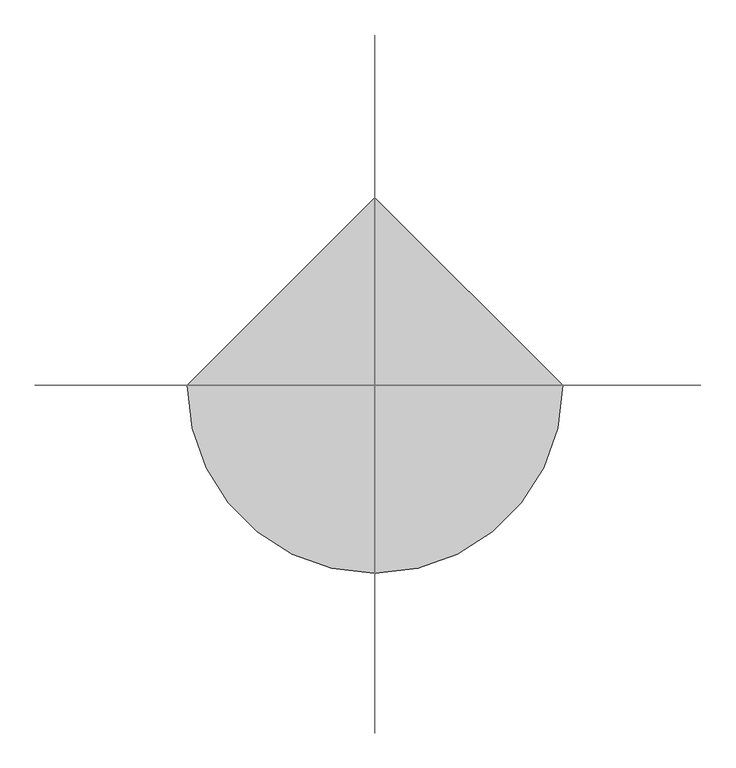
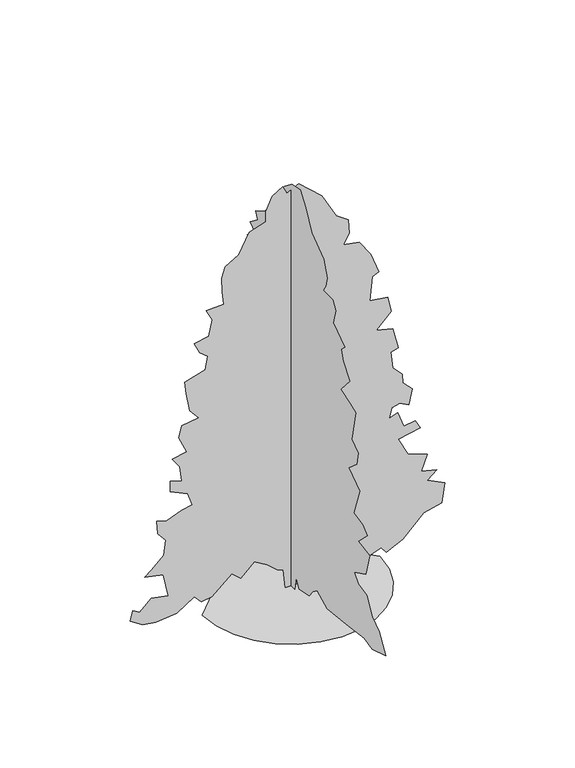
"""IFC4 building model written with IfcOpenShell, lengths in millimetres: proxy geometry, colorado spruce 26066 : colorado spruce 26066."""

from ifc_helpers import new_model, si_unit, origin, place, context, project, spatial, triangles, source, transform, mapped, element, save


def entourage_51173285(model_context):
    return source(origin(), model_context, "Body", "Tessellation", [
        triangles([(2.3e-06, 50.6216921, 3.68e-05), (9.8e-06, 78.1276076, 213.1710181), (1.43e-05, 112.5100566, 309.4405598), (1.77e-05, 236.2865403, 240.6769336), (2.27e-05, 387.5684217, 178.7885601), (2.95e-05, 559.4807118, 151.2826536), (3.74e-05, 731.8705164, 158.5998759), (3.48e-05, 752.0228474, 41.258996), (4.28e-05, 875.7995945, 123.776738), (4.61e-05, 1007.1354006, 36.9163581), (5.13e-05, 1102.7231707, 68.7649115), (5.94e-05, 1288.3895267, 61.888369), (6.59e-05, 1377.7823261, 144.4061111), (8e-05, 1570.324498, 330.0704415), (7.64e-05, 1453.423494, 385.0817639), (7.29e-05, 1350.2767376, 419.465748), (6.83e-05, 1254.1961197, 411.4393484), (7.07e-05, 1233.3757336, 522.6126134), (7.48e-05, 1260.8813221, 618.883663), (8.24e-05, 1357.1524807, 728.9063078), (7.87e-05, 1260.8813221, 749.5362259), (8.41e-05, 1336.5226353, 818.3016506), (7.99e-05, 1219.624102, 852.6830549), (7.62e-05, 1095.8474276, 914.5726639), (7.72e-05, 1032.2102509, 1041.9130743), (8.57e-05, 1192.1185135, 1086.4849903), (9.06e-05, 1260.8813221, 1148.3720558), (8.72e-05, 1171.4885954, 1169.0019739), (8.31e-05, 1020.2061871, 1258.3973167), (8.97e-05, 1130.2288319, 1313.4086391), (9.55e-05, 1139.1290154, 1494.4927895), (9.04e-05, 1013.3279005, 1512.8265541), (8.63e-05, 903.3052557, 1540.3321426), (9.07e-05, 919.5358784, 1665.6252216), (9.79e-05, 1053.5310425, 1703.3976254), (0.0001031, 1082.0933252, 1836.0212162), (9.76e-05, 972.0706804, 1815.3912254), (9.84e-05, 902.5889477, 1949.2238995), (0.0001046, 978.9464235, 2042.3148743), (0.0001028, 882.6754103, 2124.8319305), (0.0001091, 978.9464235, 2193.5973553), (0.000112, 1006.4520847, 2248.6086777), (0.0001076, 834.539831, 2358.6337933), (0.0001087, 813.9099855, 2427.3966019), (0.0001169, 951.4407623, 2496.1621719), (0.0001168, 889.5511534, 2585.5674706), (0.0001125, 752.0228474, 2647.4418915), (0.0001196, 841.4156467, 2750.5914093), (0.0001179, 745.1445608, 2839.9740349), (0.0001151, 621.3703571, 2929.3819496), (0.0001181, 614.4919979, 3039.4147682), (0.0001241, 717.6388996, 3087.5475861), (0.0001224, 642.0002026, 3142.5639954), (0.000119, 552.6049324, 3163.1888992), (0.0001267, 669.5058638, 3245.688224), (0.000124, 545.729153, 3341.9794395), (0.0001276, 580.1105936, 3410.7374519), (0.0001236, 435.7039647, 3493.2617752), (0.000122, 318.802997, 3617.0361969), (0.0001233, 241.6693149, 3775.8113892), (0.000122, 98.7569716, 3947.1090729), (0.0001198, -11.2668813, 4036.4916985), (0.0001145, -148.7964954, 4063.9999031), (0.0001065, -245.067327, 3940.2257721), (9.64e-05, -341.337886, 3747.6936287), (8.32e-05, -540.7558373, 3603.2693047), (7.6e-05, -595.7671597, 3445.1289574), (7.44e-05, -568.2614985, 3348.8374512), (7.41e-05, -533.8800579, 3286.9630302), (6.73e-05, -685.1624662, 3286.9630302), (6.27e-05, -733.2979729, 3204.4384163), (6.03e-05, -692.0382093, 3060.0396721), (4.78e-05, -884.5803812, 2929.3819496), (4.89e-05, -822.6907722, 2874.3655403), (4.43e-05, -857.07472, 2771.2160225), (3.55e-05, -967.0973648, 2640.5585907), (3.71e-05, -815.8149565, 2468.6562927), (2.85e-05, -975.0983299, 2418.8978474), (2.34e-05, -1063.3684507, 2379.2636387), (1.71e-05, -1001.4787691, 2076.6963512), (1.03e-05, -1104.6282143, 2001.0551834), (7.5e-06, -1083.9982962, 1877.2784363), (9.8e-06, -953.3432625, 1760.3800484), (-1.8e-06, -1132.1338755, 1636.6033012), (-5.6e-06, -1028.9869738, 1354.6658592), (-1.32e-05, -1180.2693821, 1327.1601254), (-1.84e-05, -1255.9105499, 1265.2730598), (-1.62e-05, -1104.6282143, 1113.9906515), (-2.56e-05, -1297.16777, 1086.4849903), (-2.93e-05, -1228.4049614, 859.5588707), (-2.37e-05, -1042.7385326, 770.1660713), (-2.89e-05, -1104.6282143, 687.6490877), (-3.62e-05, -1249.032336, 660.1434265), (-4.49e-05, -1338.4276062, 501.9827316), (-5.26e-05, -1455.3284649, 419.465748), (-6.25e-05, -1558.4753666, 240.6769336), (-5.47e-05, -1338.4276062, 171.9120176), (-4.78e-05, -1203.4697828, 202.7582816), (-3.57e-05, -909.8228811, 166.6996904), (-2.27e-05, -595.7671597, 130.6530262), (-1.29e-05, -430.7306491, 213.1710181), (-1.15e-05, -361.9677678, 158.1589326), (-1.1e-05, -300.0781407, 82.5177376), (-4.6e-06, -135.0434104, 48.1355384), (1e-07, -87.2685559, 135.4498173), (-2.7e-06, -59.4022154, 3.35e-05), (-52.2236701, 1.3e-06, 3.68e-05), (-72.8530386, -2.11e-05, 185.6651025), (-127.8648697, -2.04e-05, 206.2944756), (-224.1356831, -2.12e-05, 288.8132396), (-347.9113947, -2.09e-05, 364.4544256), (-478.5664647, 3.3e-06, 240.6769336), (-561.0834483, 2.4e-06, 316.3188827), (-753.6255838, 1.55e-05, 151.2826536), (-850.3106707, 1.89e-05, 139.1823475), (-918.659551, 1.76e-05, 213.1710181), (-1083.6960617, 2.75e-05, 103.147365), (-1283.1139767, 4.91e-05, 82.5179919), (-1406.8907238, 5.18e-05, 103.147365), (-1523.7917278, 5.2e-05, 178.7885601), (-1503.1617371, 4.7e-05, 275.0591373), (-1434.3964577, 4.68e-05, 233.8003911), (-1324.3711967, 2.42e-05, 336.9487644), (-1166.2130453, 2.07e-05, 309.4405598), (-1212.8550385, 1.19e-05, 536.5622706), (-1386.2608784, 1.56e-05, 570.7481564), (-1324.3711967, 1.16e-05, 618.883663), (-1207.4728088, 3.2e-06, 728.9063078), (-1186.8428907, -3.9e-06, 873.312973), (-1262.4841312, -5.6e-06, 962.7082432), (-1276.2382336, -1.11e-05, 1093.3607334), (-1179.9671476, -1.27e-05, 1065.8550722), (-1035.5604824, -3.42e-05, 1120.8663946), (-939.2894691, -3.8e-05, 1141.4963127), (-980.5492327, -4.23e-05, 1265.2730598), (-1145.7305019, -4.09e-05, 1342.6363609), (-1145.5831272, -4.57e-05, 1450.9368725), (-1035.5604824, -4.74e-05, 1416.5553955), (-1054.1152365, -5.34e-05, 1562.7171135), (-1124.9558252, -5.58e-05, 1664.1088898), (-987.4249758, -6.12e-05, 1691.6146236), (-1063.0661436, -6.63e-05, 1856.6484455), (-1035.5604824, -7.2e-05, 1966.6737064), (-877.402331, -9.27e-05, 1994.179295), (-959.9193146, -9.46e-05, 2090.4504536), (-994.3007915, -0.0001019, 2276.1142662), (-1008.0548212, -0.0001067, 2393.0152702), (-815.512722, -0.0001152, 2454.9021904), (-788.0070608, -0.0001215, 2578.6841698), (-863.6482286, -0.000122, 2640.5585907), (-918.659551, -0.0001253, 2750.5914093), (-778.8249178, -0.0001453, 2774.1370651), (-746.7472973, -0.0001532, 2929.3819496), (-801.7586197, -0.0001565, 3039.4147682), (-636.7246525, -0.0001617, 3046.2727798), (-650.4762114, -0.0001671, 3176.9302116), (-657.3544979, -0.0001731, 3314.4712349), (-622.9705502, -0.0001787, 3417.6207527), (-495.5108156, -0.0002008, 3495.9796326), (-396.0469377, -0.0002122, 3685.7939186), (-237.8885137, -0.0002191, 3733.9270271), (-237.8885137, -0.0002237, 3837.0762543), (-176.0001583, -0.0002314, 3967.7339767), (-79.7295811, -0.000237, 4029.6083977), (-38.4705851, -0.0002349, 3953.9670845), (71.553068, -0.0002554, 4008.9834938), (291.5996066, -0.000253, 3809.5680496), (429.1304561, -0.0002313, 3562.0197876), (546.0314238, -0.0002458, 3479.4951736), (552.9072032, -0.0002251, 3341.9794395), (497.8958808, -0.0002192, 3245.688224), (649.1782528, -0.0002225, 3218.2053085), (759.2008976, -0.0002187, 3060.0396721), (834.8420654, -0.000212, 2860.6242279), (772.2870174, -0.0002087, 2828.0866791), (745.4493387, -0.0001977, 2599.3090736), (917.359049, -0.0002016, 2571.800869), (951.7430695, -0.0001958, 2420.5208588), (807.3364769, -0.0001854, 2282.9926254), (965.4946283, -0.0001882, 2241.7327892), (1020.5084942, -0.0001656, 2028.5607719), (944.8647102, -0.0001627, 2014.8092857), (965.4946283, -0.000156, 1849.7727024), (1056.4342083, -0.0001542, 1750.4358879), (1061.7657143, -0.0001505, 1664.1088898), (1151.1609844, -0.0001492, 1574.7136196), (1116.7770367, -0.0001414, 1423.4311386), (1034.2600531, -0.0001411, 1471.5667179), (958.6188126, -0.0001379, 1450.9368725), (931.1131514, -0.0001328, 1354.6658592), (1013.630135, -0.0001365, 1382.1714478), (1068.6414574, -0.0001311, 1224.0132236), (1178.6666456, -0.0001353, 1244.6432144), (1226.8021523, -0.0001327, 1155.2478716), (1020.5084942, -0.0001247, 1113.9906515), (1109.9012209, -0.0001046, 935.2000385), (1295.567577, -0.0001218, 866.4371572), (1236.1544884, -9.85e-05, 715.1572924), (1384.9603764, -0.0001014, 680.7708012), (1295.567577, -9.54e-05, 605.129597), (1460.6015442, -9.66e-05, 522.6126134), (1433.0959557, -8.72e-05, 330.0704415), (1261.1836292, -8.02e-05, 288.8132396), (1062.7105694, -6.57e-05, 95.753176), (903.6074902, -4.28e-05, 20.6293708), (855.4719835, -4.42e-05, 82.5177376), (674.9694111, -3.6e-05, 21.2873589), (484.1417785, -3e-05, 13.7529317), (408.5005743, -3.08e-05, 82.5177376), (236.5885567, -2.85e-05, 144.4061111), (74.3397029, -2.22e-05, 111.1694498), (57.799983, -1.67e-05, 3.35e-05), (-841.6823456, -4.7e-06, 6.03e-05), (-819.4294161, -192.8576323, 5.39e-05), (-756.0589382, -369.9662258, 4.68e-05), (-656.640806, -526.2524348, 3.91e-05), (-526.2524348, -656.640806, 3.14e-05), (-369.9662258, -756.0589382, 2.37e-05), (-192.8576323, -819.4294161, 1.66e-05), (3.68e-05, -841.6823456, 1.02e-05), (192.8576323, -819.4294161, 5.1e-06), (369.9662258, -756.0589382, 1.7e-06), (526.2524348, -656.640806, 0.0), (656.640806, -526.2524348, 0.0), (756.0589382, -369.9662258, 1.7e-06), (819.4294161, -192.8576323, 5.1e-06), (841.6823456, 7.8e-05, 1.02e-05), (-0.0001104, 841.6823456, 6.03e-05)], [[26, 27, 28], [21, 22, 23], [19, 20, 21], [51, 52, 53], [7, 8, 9], [35, 36, 37], [13, 14, 15], [34, 35, 37], [54, 55, 56], [72, 73, 74], [95, 96, 97], [88, 89, 90], [44, 45, 46], [86, 87, 88], [85, 86, 88], [51, 53, 54], [44, 46, 47], [88, 90, 91], [13, 15, 16], [13, 16, 17], [38, 39, 40], [25, 26, 28], [25, 28, 29], [47, 48, 49], [56, 57, 58], [30, 31, 32], [29, 30, 32], [41, 42, 43], [40, 41, 43], [106, 1, 2], [105, 106, 2], [75, 76, 77], [94, 95, 97], [94, 97, 98], [78, 79, 80], [83, 84, 85], [29, 32, 33], [103, 104, 105], [12, 13, 17], [11, 12, 17], [77, 78, 80], [102, 103, 105], [62, 63, 64], [80, 81, 82], [80, 82, 83], [61, 62, 64], [61, 64, 65], [60, 61, 65], [59, 60, 65], [69, 70, 71], [69, 71, 72], [94, 98, 99], [93, 94, 99], [92, 93, 99], [92, 99, 100], [91, 92, 100], [91, 100, 101], [47, 49, 50], [9, 10, 11], [9, 11, 17], [9, 17, 18], [7, 9, 18], [59, 65, 66], [59, 66, 67], [59, 67, 68], [59, 68, 69], [58, 59, 69], [56, 58, 69], [54, 56, 69], [54, 69, 72], [51, 54, 72], [50, 51, 72], [50, 72, 74], [50, 74, 75], [50, 75, 77], [47, 50, 77], [44, 47, 77], [43, 44, 77], [40, 43, 77], [40, 77, 80], [40, 80, 83], [38, 40, 83], [38, 83, 85], [37, 38, 85], [34, 37, 85], [33, 34, 85], [29, 33, 85], [25, 29, 85], [25, 85, 88], [25, 88, 91], [25, 91, 101], [25, 101, 102], [24, 25, 102], [23, 24, 102], [21, 23, 102], [105, 2, 3], [102, 105, 3], [21, 102, 3], [21, 3, 4], [21, 4, 5], [21, 5, 6], [21, 6, 7], [21, 7, 18], [19, 21, 18], [125, 126, 127], [198, 199, 200], [153, 154, 155], [139, 140, 141], [130, 131, 132], [120, 121, 122], [119, 120, 122], [186, 187, 188], [136, 137, 138], [135, 136, 138], [150, 151, 152], [193, 194, 195], [192, 193, 195], [125, 127, 128], [180, 181, 182], [163, 164, 165], [185, 186, 188], [196, 197, 198], [190, 191, 192], [111, 112, 113], [212, 107, 108], [211, 212, 108], [173, 174, 175], [149, 150, 152], [179, 180, 182], [129, 130, 132], [146, 147, 148], [204, 205, 206], [200, 201, 202], [200, 202, 203], [162, 163, 165], [190, 192, 195], [165, 166, 167], [118, 119, 122], [118, 122, 123], [118, 123, 124], [117, 118, 124], [116, 117, 124], [176, 177, 178], [176, 178, 179], [129, 132, 133], [185, 188, 189], [142, 143, 144], [141, 142, 144], [161, 162, 165], [161, 165, 167], [161, 167, 168], [116, 124, 125], [145, 146, 148], [144, 145, 148], [114, 115, 116], [113, 114, 116], [113, 116, 125], [113, 125, 128], [113, 128, 129], [113, 129, 133], [113, 133, 134], [111, 113, 134], [168, 169, 170], [168, 170, 171], [161, 168, 171], [160, 161, 171], [159, 160, 171], [158, 159, 171], [157, 158, 171], [156, 157, 171], [155, 156, 171], [171, 172, 173], [171, 173, 175], [155, 171, 175], [155, 175, 176], [153, 155, 176], [152, 153, 176], [149, 152, 176], [149, 176, 179], [148, 149, 179], [144, 148, 179], [144, 179, 182], [144, 182, 183], [141, 144, 183], [139, 141, 183], [138, 139, 183], [135, 138, 183], [134, 135, 183], [111, 134, 183], [110, 111, 183], [110, 183, 184], [110, 184, 185], [110, 185, 189], [110, 189, 190], [110, 190, 195], [109, 110, 195], [108, 109, 195], [211, 108, 195], [210, 211, 195], [210, 195, 196], [209, 210, 196], [209, 196, 198], [208, 209, 198], [207, 208, 198], [206, 207, 198], [204, 206, 198], [203, 204, 198], [200, 203, 198], [227, 228, 213], [226, 227, 213], [226, 213, 214], [225, 226, 214], [225, 214, 215], [225, 215, 216], [224, 225, 216], [223, 224, 216], [223, 216, 217], [223, 217, 218], [223, 218, 219], [223, 219, 220], [223, 220, 221], [223, 221, 222]], closed=False),
    ])


if __name__ == "__main__":
    model = new_model("IFC4")
    model_context = context("Model", 3, world=origin())
    ifc_project = project(units=[si_unit("LENGTHUNIT", "METRE", prefix="MILLI")], contexts=[model_context])
    site = spatial("IfcSite", under=ifc_project)
    building = spatial("IfcBuilding", under=site)
    placement = place(None, origin())
    entourage_shape = entourage_51173285(model_context)
    element("IfcBuildingElementProxy", 1, Name="colorado spruce 26066 : colorado spruce 26066", ObjectType="colorado spruce 26066 : colorado spruce 26066", at=placement, inside=building, context=model_context, shape_type="MappedRepresentation", body=[
        mapped(entourage_shape, transform((0.0, 0.0, 0.0), x_axis=(1.0, 0.0, 0.0), y_axis=(0.0, 1.0, 0.0), z_axis=(0.0, 0.0, 1.0))),
    ])
    save(model, "model.ifc")

# Revit data of these elements
# Type "colorado spruce 26066 : colorado spruce 26066"
#   built-in parameter 1005195 = "RPC-16-G0M4-N9PX-U6TN-C000-ST1L-LVER-AU"
#   Height = 0
